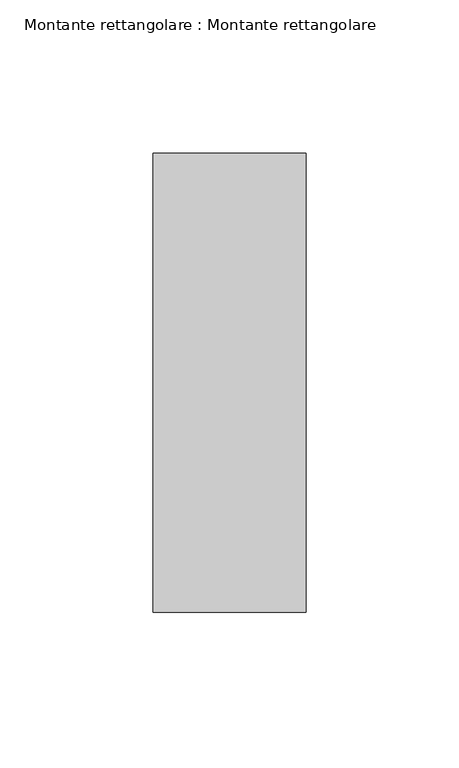
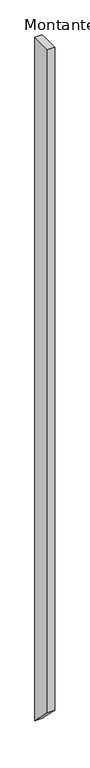
"""IFC4 building model written with IfcOpenShell, lengths in millimetres: member geometry, Montante rettangolare : Montante rettangolare."""

from ifc_helpers import new_model, si_unit, frame, origin, place, context, project, spatial, polyline, outline, extrude, source, transform, mapped, element, save


def montante_rettangolare_montante_rettangolare_c5eda454(model_context):
    return source(origin(), model_context, "Body", "SweptSolid", [
        extrude(outline(polyline([(-75.0, 0.0), (75.0, 0.0), (75.0, -4995.0), (-75.0, -4845.0), (-75.0, 0.0)])), frame((-50.0, 0.0, 0.0), z_axis=(1.0, 0.0, 0.0), x_axis=(0.0, 1.0, 0.0)), (0.0, 0.0, 1.0), 50.0),
    ])


if __name__ == "__main__":
    model = new_model("IFC4")
    model_context = context("Model", 3, world=origin())
    ifc_project = project(units=[si_unit("LENGTHUNIT", "METRE", prefix="MILLI")], contexts=[model_context])
    site = spatial("IfcSite", under=ifc_project)
    building = spatial("IfcBuilding", under=site)
    placement = place(None, origin())
    montante_rettangolare_montante_rettangolare_shape = montante_rettangolare_montante_rettangolare_c5eda454(model_context)
    element("IfcMember", 1, ObjectType="Montante rettangolare : Montante rettangolare", at=placement, inside=building, context=model_context, shape_type="MappedRepresentation", body=[
        mapped(montante_rettangolare_montante_rettangolare_shape, transform((0.0, 0.0, 0.0), x_axis=(1.0, 0.0, 0.0), y_axis=(0.0, 1.0, 0.0), z_axis=(0.0, 0.0, 1.0))),
    ])
    save(model, "model.ifc")

# Revit data of these elements
# Type "Montante rettangolare : Montante rettangolare"
#   built-in parameter 1007304 = 0.492126 (stored number, unit not read)
#   built-in parameter 1007301 = 0.082021 (stored number, unit not read)
#   built-in parameter 1007300 = 0.082021 (stored number, unit not read)
# Element 1 (IfcMember, "Montante rettangolare : Montante rettangolare")
#   Materials on its faces: "Acciaio"
# Materials
#   "Acciaio": class "Metallo", colour RGB 247 247 247, transparency 0, Description = "Acciaio, finitura zigrinata", Cost = 0
